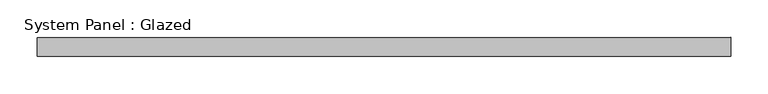
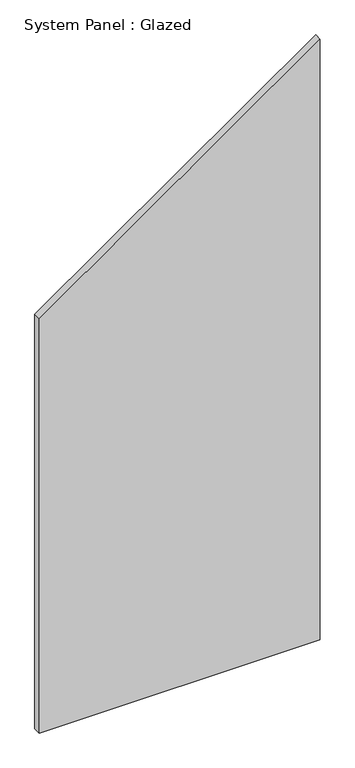
"""IFC4 building model written with IfcOpenShell, lengths in millimetres: plate geometry, System Panel : Glazed."""

from ifc_helpers import new_model, si_unit, frame, origin, place, context, project, spatial, polyline, outline, extrude, source, transform, mapped, element, save


def system_panel_glazed_7be6faa8(model_context):
    return source(origin(), model_context, "Body", "SweptSolid", [
        extrude(outline(polyline([(0.0, -462.5), (0.0, 462.5), (2089.4282315, 462.5), (1441.7362587, -462.5), (0.0, -462.5)])), frame((0.0, 24.5, 0.0), z_axis=(0.0, 1.0, 0.0), x_axis=(0.0, 0.0, 1.0)), (0.0, 0.0, 1.0), 25.0),
    ])


if __name__ == "__main__":
    model = new_model("IFC4")
    model_context = context("Model", 3, world=origin())
    ifc_project = project(units=[si_unit("LENGTHUNIT", "METRE", prefix="MILLI")], contexts=[model_context])
    site = spatial("IfcSite", under=ifc_project)
    building = spatial("IfcBuilding", under=site)
    placement = place(None, origin())
    system_panel_glazed_shape = system_panel_glazed_7be6faa8(model_context)
    element("IfcPlate", 1, ObjectType="System Panel : Glazed", at=placement, inside=building, context=model_context, shape_type="MappedRepresentation", body=[
        mapped(system_panel_glazed_shape, transform((0.0, 0.0, 0.0), x_axis=(1.0, 0.0, 0.0), y_axis=(0.0, 1.0, 0.0), z_axis=(0.0, 0.0, 1.0))),
    ])
    save(model, "model.ifc")

# Revit data of these elements
# Type "System Panel : Glazed"
#   Construction Type Id = "GSP4R"
#   Analytic Construction = "1/8 in Pilkington single glazing"
#   Visual Light Transmittance = 0.9
#   Solar Heat Gain Coefficient = 0.86
#   Heat Transfer Coefficient (U) = 6.7069 W/(m²·K)
#   Define Thermal Properties by = 1
# Element 1 (IfcPlate, "System Panel : Glazed")
#   Materials on its faces: "Glass"
# Materials
#   "Glass": class "Glass", colour RGB 0 128 192, transparency 0.9, Description = "Soda Lime Glass", Cost = 0
